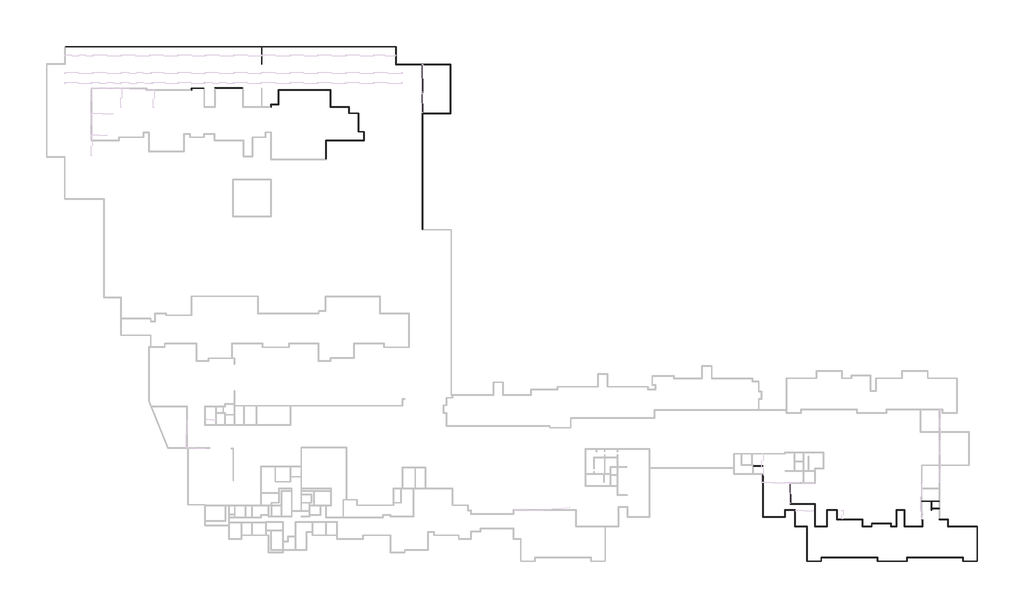
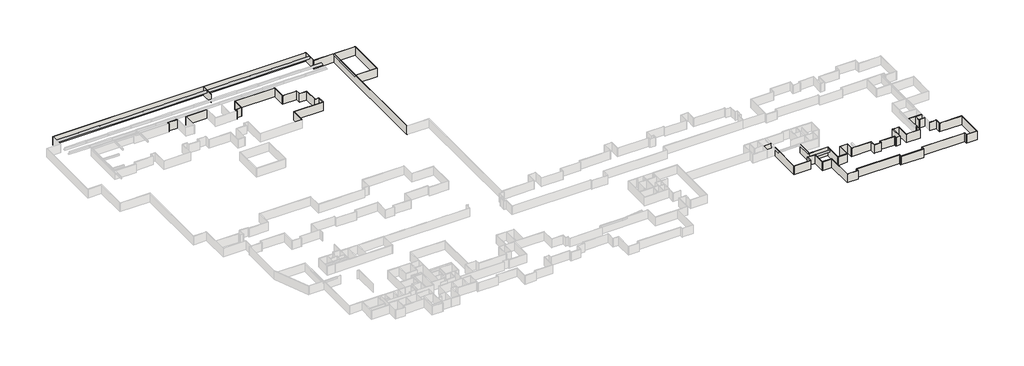
# One storey, part 6 of 8: 67 walls.
"""IFC4 building model written with IfcOpenShell, lengths in millimetres."""

from ifc_helpers import new_model, si_unit, origin, origin_with_axes, place, context, project, spatial, polyline, outline, extrude, faceted_brep, element, save

model = new_model("IFC4")

# Units and contexts
model_context = context("Model", 3, world=origin())
ifc_project = project(units=[si_unit("LENGTHUNIT", "METRE", prefix="MILLI")], contexts=[model_context])

# Site, building, storey
site = spatial("IfcSite", under=ifc_project)
building = spatial("IfcBuilding", under=site)
storey = spatial("IfcBuildingStorey", under=building, Name="户型图", Elevation=0.0)

# Walls
placement = place(None, origin())
element("IfcWall", 1, ObjectType="所有墙体", at=placement, inside=storey, context=model_context, shape_type="Brep", body=[
    faceted_brep([(258613.8534901, 37656.7427445, 0.0), (258613.8534901, 25547.5338444, 0.0), (258613.8534901, 25547.5338444, 3300.0), (258613.8534901, 37656.7427445, 3300.0), (258733.8534901, 37656.7427445, 0.0), (258733.8534901, 37656.7427445, 3300.0), (258733.8534901, 25667.5338444, 3300.0), (258733.8534901, 25547.5338444, 3300.0), (258733.8534901, 25547.5338444, 0.0), (258733.8534901, 25667.5338444, 0.0)], [[[0, 1, 2, 3]], [[4, 5, 6, 7, 8, 9]], [[1, 0, 4, 9, 8]], [[3, 2, 7, 6, 5]], [[0, 3, 5, 4]], [[2, 1, 8, 7]]]),
])
element("IfcWall", 2, ObjectType="所有墙体", at=placement, inside=storey, context=model_context, shape_type="Brep", body=[
    faceted_brep([(258733.8534901, 25547.5338444, 0.0), (264932.3033606, 25547.5338444, 0.0), (264932.3033606, 25547.5338444, 3300.0), (258733.8534901, 25547.5338444, 3300.0), (258733.8534901, 25667.5338444, 0.0), (258733.8534901, 25667.5338444, 3300.0), (264812.3033606, 25667.5338444, 3300.0), (264932.3033606, 25667.5338444, 3300.0), (264932.3033606, 25667.5338444, 0.0), (264812.3033606, 25667.5338444, 0.0)], [[[0, 1, 2, 3]], [[4, 5, 6, 7, 8, 9]], [[1, 0, 4, 9, 8]], [[3, 2, 7, 6, 5]], [[0, 3, 5, 4]], [[2, 1, 8, 7]]]),
])
element("IfcWall", 3, ObjectType="所有墙体", at=placement, inside=storey, context=model_context, shape_type="Brep", body=[
    faceted_brep([(264932.3033606, 25667.5338444, 0.0), (264932.3033606, 27556.847508, 0.0), (264932.3033606, 27676.847508, 0.0), (264932.3033606, 27676.847508, 3300.0), (264932.3033606, 27556.847508, 3300.0), (264932.3033606, 25667.5338444, 3300.0), (264812.3033606, 25667.5338444, 0.0), (264812.3033606, 25667.5338444, 3300.0), (264812.3033606, 27676.847508, 3300.0), (264812.3033606, 27676.847508, 0.0)], [[[0, 1, 2, 3, 4, 5]], [[6, 7, 8, 9]], [[2, 1, 0, 6, 9]], [[5, 4, 3, 8, 7]], [[0, 5, 7, 6]], [[3, 2, 9, 8]]]),
])
element("IfcWall", 4, ObjectType="所有墙体", at=placement, inside=storey, context=model_context, shape_type="Brep", body=[
    faceted_brep([(264932.3033606, 27556.847508, 0.0), (267613.3412105, 27556.847508, 0.0), (267733.3412105, 27556.847508, 0.0), (267733.3412105, 27556.847508, 3300.0), (267613.3412105, 27556.847508, 3300.0), (264932.3033606, 27556.847508, 3300.0), (264932.3033606, 27676.847508, 0.0), (264932.3033606, 27676.847508, 3300.0), (267733.3412105, 27676.847508, 3300.0), (267733.3412105, 27676.847508, 0.0)], [[[0, 1, 2, 3, 4, 5]], [[6, 7, 8, 9]], [[2, 1, 0, 6, 9]], [[5, 4, 3, 8, 7]], [[0, 5, 7, 6]], [[3, 2, 9, 8]]]),
])
element("IfcWall", 5, ObjectType="所有墙体", at=placement, inside=storey, context=model_context, shape_type="Brep", body=[
    faceted_brep([(267613.3412105, 27556.847508, 0.0), (267613.3412105, 22947.648549, 0.0), (267613.3412105, 22947.648549, 3300.0), (267613.3412105, 27556.847508, 3300.0), (267733.3412105, 27556.847508, 0.0), (267733.3412105, 27556.847508, 3300.0), (267733.3412105, 23067.648549, 3300.0), (267733.3412105, 22947.648549, 3300.0), (267733.3412105, 22947.648549, 0.0), (267733.3412105, 23067.648549, 0.0)], [[[0, 1, 2, 3]], [[4, 5, 6, 7, 8, 9]], [[1, 0, 4, 9, 8]], [[3, 2, 7, 6, 5]], [[0, 3, 5, 4]], [[2, 1, 8, 7]]]),
])
element("IfcWall", 6, ObjectType="所有墙体", at=placement, inside=storey, context=model_context, shape_type="Brep", body=[
    faceted_brep([(267733.3412105, 22947.648549, 0.0), (271063.0918563, 22947.648549, 0.0), (271183.0918563, 22947.648549, 0.0), (271183.0918563, 22947.648549, 3300.0), (271063.0918563, 22947.648549, 3300.0), (267733.3412105, 22947.648549, 3300.0), (267733.3412105, 23067.648549, 0.0), (267733.3412105, 23067.648549, 3300.0), (271183.0918563, 23067.648549, 3300.0), (271183.0918563, 23067.648549, 0.0)], [[[0, 1, 2, 3, 4, 5]], [[6, 7, 8, 9]], [[2, 1, 0, 6, 9]], [[5, 4, 3, 8, 7]], [[0, 5, 7, 6]], [[3, 2, 9, 8]]]),
])
element("IfcWall", 7, ObjectType="所有墙体", at=placement, inside=storey, context=model_context, shape_type="Brep", body=[
    faceted_brep([(271063.0918563, 22947.648549, 0.0), (271063.0918563, 13147.6884452, 0.0), (271063.0918563, 13147.6884452, 3300.0), (271063.0918563, 22947.648549, 3300.0), (271183.0918563, 22947.648549, 0.0), (271183.0918563, 22947.648549, 3300.0), (271183.0918563, 13267.6884452, 3300.0), (271183.0918563, 13147.6884452, 3300.0), (271183.0918563, 13147.6884452, 0.0), (271183.0918563, 13267.6884452, 0.0)], [[[0, 1, 2, 3]], [[4, 5, 6, 7, 8, 9]], [[1, 0, 4, 9, 8]], [[3, 2, 7, 6, 5]], [[0, 3, 5, 4]], [[2, 1, 8, 7]]]),
])
element("IfcWall", 8, ObjectType="所有墙体", at=placement, inside=storey, context=model_context, shape_type="Brep", body=[
    faceted_brep([(271183.0918563, 13147.6884452, 0.0), (275183.1173563, 13147.6884452, 0.0), (275183.1173563, 13147.6884452, 3300.0), (271183.0918563, 13147.6884452, 3300.0), (271183.0918563, 13267.6884452, 0.0), (271183.0918563, 13267.6884452, 3300.0), (275063.1173563, 13267.6884452, 3300.0), (275183.1173563, 13267.6884452, 3300.0), (275183.1173563, 13267.6884452, 0.0), (275063.1173563, 13267.6884452, 0.0)], [[[0, 1, 2, 3]], [[4, 5, 6, 7, 8, 9]], [[1, 0, 4, 9, 8]], [[3, 2, 7, 6, 5]], [[0, 3, 5, 4]], [[2, 1, 8, 7]]]),
])
element("IfcWall", 9, ObjectType="所有墙体", at=placement, inside=storey, context=model_context, shape_type="Brep", body=[
    faceted_brep([(275183.1173563, 13267.6884452, 0.0), (275183.1173563, 14147.2784493, 0.0), (275183.1173563, 14267.2784493, 0.0), (275183.1173563, 14267.2784493, 3300.0), (275183.1173563, 14147.2784493, 3300.0), (275183.1173563, 13267.6884452, 3300.0), (275063.1173563, 13267.6884452, 0.0), (275063.1173563, 13267.6884452, 3300.0), (275063.1173563, 14267.2784493, 3300.0), (275063.1173563, 14267.2784493, 0.0)], [[[0, 1, 2, 3, 4, 5]], [[6, 7, 8, 9]], [[2, 1, 0, 6, 9]], [[5, 4, 3, 8, 7]], [[0, 5, 7, 6]], [[3, 2, 9, 8]]]),
])
element("IfcWall", 10, ObjectType="所有墙体", at=placement, inside=storey, context=model_context, shape_type="Brep", body=[
    faceted_brep([(275183.1173563, 14147.2784493, 0.0), (290862.8910266, 14147.2784493, 0.0), (290982.8910266, 14147.2784493, 0.0), (290982.8910266, 14147.2784493, 3300.0), (290862.8910266, 14147.2784493, 3300.0), (275183.1173563, 14147.2784493, 3300.0), (275183.1173563, 14267.2784493, 0.0), (275183.1173563, 14267.2784493, 3300.0), (290982.8910266, 14267.2784493, 3300.0), (290982.8910266, 14267.2784493, 0.0)], [[[0, 1, 2, 3, 4, 5]], [[6, 7, 8, 9]], [[2, 1, 0, 6, 9]], [[5, 4, 3, 8, 7]], [[0, 5, 7, 6]], [[3, 2, 9, 8]]]),
])
element("IfcWall", 11, ObjectType="所有墙体", at=placement, inside=storey, context=model_context, shape_type="Brep", body=[
    faceted_brep([(290862.8910266, 14147.2784493, 0.0), (290862.8910266, 13147.6884452, 0.0), (290862.8910266, 13147.6884452, 3300.0), (290862.8910266, 14147.2784493, 3300.0), (290982.8910266, 14147.2784493, 0.0), (290982.8910266, 14147.2784493, 3300.0), (290982.8910266, 13267.6884452, 3300.0), (290982.8910266, 13147.6884452, 3300.0), (290982.8910266, 13147.6884452, 0.0), (290982.8910266, 13267.6884452, 0.0)], [[[0, 1, 2, 3]], [[4, 5, 6, 7, 8, 9]], [[1, 0, 4, 9, 8]], [[3, 2, 7, 6, 5]], [[0, 3, 5, 4]], [[2, 1, 8, 7]]]),
])
element("IfcWall", 12, ObjectType="所有墙体", at=placement, inside=storey, context=model_context, shape_type="Brep", body=[
    faceted_brep([(290982.8910266, 13147.6884452, 0.0), (299283.1811417, 13147.6884452, 0.0), (299283.1811417, 13147.6884452, 3300.0), (290982.8910266, 13147.6884452, 3300.0), (290982.8910266, 13267.6884452, 0.0), (290982.8910266, 13267.6884452, 3300.0), (299163.1811417, 13267.6884452, 3300.0), (299283.1811417, 13267.6884452, 3300.0), (299283.1811417, 13267.6884452, 0.0), (299163.1811417, 13267.6884452, 0.0)], [[[0, 1, 2, 3]], [[4, 5, 6, 7, 8, 9]], [[1, 0, 4, 9, 8]], [[3, 2, 7, 6, 5]], [[0, 3, 5, 4]], [[2, 1, 8, 7]]]),
])
element("IfcWall", 13, ObjectType="所有墙体", at=placement, inside=storey, context=model_context, shape_type="Brep", body=[
    faceted_brep([(299283.1811417, 13267.6884452, 0.0), (299283.1811417, 14147.2784493, 0.0), (299283.1811417, 14267.2784493, 0.0), (299283.1811417, 14267.2784493, 3300.0), (299283.1811417, 14147.2784493, 3300.0), (299283.1811417, 13267.6884452, 3300.0), (299163.1811417, 13267.6884452, 0.0), (299163.1811417, 13267.6884452, 3300.0), (299163.1811417, 14267.2784493, 3300.0), (299163.1811417, 14267.2784493, 0.0)], [[[0, 1, 2, 3, 4, 5]], [[6, 7, 8, 9]], [[2, 1, 0, 6, 9]], [[5, 4, 3, 8, 7]], [[0, 5, 7, 6]], [[3, 2, 9, 8]]]),
])
element("IfcWall", 14, ObjectType="所有墙体", at=placement, inside=storey, context=model_context, shape_type="Brep", body=[
    faceted_brep([(299283.1811417, 14147.2784493, 0.0), (314962.8909977, 14147.2784493, 0.0), (315082.8909977, 14147.2784493, 0.0), (315082.8909977, 14147.2784493, 3300.0), (314962.8909977, 14147.2784493, 3300.0), (299283.1811417, 14147.2784493, 3300.0), (299283.1811417, 14267.2784493, 0.0), (299283.1811417, 14267.2784493, 3300.0), (315082.8909977, 14267.2784493, 3300.0), (315082.8909977, 14267.2784493, 0.0)], [[[0, 1, 2, 3, 4, 5]], [[6, 7, 8, 9]], [[2, 1, 0, 6, 9]], [[5, 4, 3, 8, 7]], [[0, 5, 7, 6]], [[3, 2, 9, 8]]]),
])
element("IfcWall", 15, ObjectType="所有墙体", at=placement, inside=storey, context=model_context, shape_type="Brep", body=[
    faceted_brep([(314962.8909977, 14147.2784493, 0.0), (314962.8909977, 13147.6884452, 0.0), (314962.8909977, 13147.6884452, 3300.0), (314962.8909977, 14147.2784493, 3300.0), (315082.8909977, 14147.2784493, 0.0), (315082.8909977, 14147.2784493, 3300.0), (315082.8909977, 13267.6884452, 3300.0), (315082.8909977, 13147.6884452, 3300.0), (315082.8909977, 13147.6884452, 0.0), (315082.8909977, 13267.6884452, 0.0)], [[[0, 1, 2, 3]], [[4, 5, 6, 7, 8, 9]], [[1, 0, 4, 9, 8]], [[3, 2, 7, 6, 5]], [[0, 3, 5, 4]], [[2, 1, 8, 7]]]),
])
element("IfcWall", 16, ObjectType="所有墙体", at=placement, inside=storey, context=model_context, shape_type="Brep", body=[
    faceted_brep([(315082.8909977, 13147.6884452, 0.0), (319083.2156356, 13147.6884452, 0.0), (319083.2156356, 13147.6884452, 3300.0), (315082.8909977, 13147.6884452, 3300.0), (315082.8909977, 13267.6884452, 0.0), (315082.8909977, 13267.6884452, 3300.0), (318963.2156356, 13267.6884452, 3300.0), (319083.2156356, 13267.6884452, 3300.0), (319083.2156356, 13267.6884452, 0.0), (318963.2156356, 13267.6884452, 0.0)], [[[0, 1, 2, 3]], [[4, 5, 6, 7, 8, 9]], [[1, 0, 4, 9, 8]], [[3, 2, 7, 6, 5]], [[0, 3, 5, 4]], [[2, 1, 8, 7]]]),
])
element("IfcWall", 17, ObjectType="所有墙体", at=placement, inside=storey, context=model_context, shape_type="Brep", body=[
    faceted_brep([(319083.2156356, 13267.6884452, 0.0), (319083.2156356, 23067.648549, 0.0), (319083.2156356, 23067.648549, 3300.0), (319083.2156356, 13267.6884452, 3300.0), (318963.2156356, 13267.6884452, 0.0), (318963.2156356, 13267.6884452, 3300.0), (318963.2156356, 22947.648549, 3300.0), (318963.2156356, 23067.648549, 3300.0), (318963.2156356, 23067.648549, 0.0), (318963.2156356, 22947.648549, 0.0)], [[[0, 1, 2, 3]], [[4, 5, 6, 7, 8, 9]], [[1, 0, 4, 9, 8]], [[3, 2, 7, 6, 5]], [[0, 3, 5, 4]], [[2, 1, 8, 7]]]),
])
element("IfcWall", 18, ObjectType="所有墙体", at=placement, inside=storey, context=model_context, shape_type="Brep", body=[
    faceted_brep([(318963.2156356, 23067.648549, 0.0), (310883.5691593, 23067.648549, 0.0), (310763.5691593, 23067.648549, 0.0), (310763.5691593, 23067.648549, 3300.0), (310883.5691593, 23067.648549, 3300.0), (318963.2156356, 23067.648549, 3300.0), (318963.2156356, 22947.648549, 0.0), (318963.2156356, 22947.648549, 3300.0), (310763.5691593, 22947.648549, 3300.0), (310763.5691593, 22947.648549, 0.0)], [[[0, 1, 2, 3, 4, 5]], [[6, 7, 8, 9]], [[2, 1, 0, 6, 9]], [[5, 4, 3, 8, 7]], [[0, 5, 7, 6]], [[3, 2, 9, 8]]]),
])
element("IfcWall", 19, ObjectType="所有墙体", at=placement, inside=storey, context=model_context, shape_type="Brep", body=[
    faceted_brep([(310883.5691593, 23067.648549, 0.0), (310883.5691593, 25066.2785565, 0.0), (310883.5691593, 25066.2785565, 3300.0), (310883.5691593, 23067.648549, 3300.0), (310763.5691593, 23067.648549, 0.0), (310763.5691593, 23067.648549, 3300.0), (310763.5691593, 24946.2785565, 3300.0), (310763.5691593, 25066.2785565, 3300.0), (310763.5691593, 25066.2785565, 0.0), (310763.5691593, 24946.2785565, 0.0)], [[[0, 1, 2, 3]], [[4, 5, 6, 7, 8, 9]], [[1, 0, 4, 9, 8]], [[3, 2, 7, 6, 5]], [[0, 3, 5, 4]], [[2, 1, 8, 7]]]),
])
element("IfcWall", 20, ObjectType="所有墙体", at=placement, inside=storey, context=model_context, shape_type="Brep", body=[
    faceted_brep([(310763.5691593, 25066.2785565, 0.0), (308483.5691593, 25066.2785565, 0.0), (308363.5691593, 25066.2785565, 0.0), (308363.5691593, 25066.2785565, 3300.0), (308483.5691593, 25066.2785565, 3300.0), (310763.5691593, 25066.2785565, 3300.0), (310763.5691593, 24946.2785565, 0.0), (310763.5691593, 24946.2785565, 3300.0), (308363.5691593, 24946.2785565, 3300.0), (308363.5691593, 24946.2785565, 0.0)], [[[0, 1, 2, 3, 4, 5]], [[6, 7, 8, 9]], [[2, 1, 0, 6, 9]], [[5, 4, 3, 8, 7]], [[0, 5, 7, 6]], [[3, 2, 9, 8]]]),
])
element("IfcWall", 21, ObjectType="所有墙体", at=placement, inside=storey, context=model_context, shape_type="Brep", body=[
    faceted_brep([(162933.8477327, 106576.635667, 0.0), (162933.8477327, 139156.635667, 0.0), (162933.8477327, 139276.635667, 0.0), (162933.8477327, 153006.6496336, 0.0), (162933.8477327, 153006.6496336, 3300.0), (162933.8477327, 139276.635667, 3300.0), (162933.8477327, 139156.635667, 3300.0), (162933.8477327, 106576.635667, 3300.0), (162813.8477327, 106576.635667, 0.0), (162813.8477327, 106576.635667, 3300.0), (162813.8477327, 153006.6496336, 3300.0), (162813.8477327, 153006.6496336, 0.0)], [[[0, 1, 2, 3, 4, 5, 6, 7]], [[8, 9, 10, 11]], [[3, 2, 1, 0, 8, 11]], [[7, 6, 5, 4, 10, 9]], [[0, 7, 9, 8]], [[4, 3, 11, 10]]]),
])
element("IfcWall", 22, ObjectType="所有墙体", at=placement, inside=storey, context=model_context, shape_type="Brep", body=[
    faceted_brep([(162933.8477327, 139156.635667, 0.0), (170833.8477327, 139156.635667, 0.0), (170833.8477327, 139156.635667, 3300.0), (162933.8477327, 139156.635667, 3300.0), (162933.8477327, 139276.635667, 0.0), (162933.8477327, 139276.635667, 3300.0), (170713.8477327, 139276.635667, 3300.0), (170833.8477327, 139276.635667, 3300.0), (170833.8477327, 139276.635667, 0.0), (170713.8477327, 139276.635667, 0.0)], [[[0, 1, 2, 3]], [[4, 5, 6, 7, 8, 9]], [[1, 0, 4, 9, 8]], [[3, 2, 7, 6, 5]], [[0, 3, 5, 4]], [[2, 1, 8, 7]]]),
])
element("IfcWall", 23, ObjectType="所有墙体", at=placement, inside=storey, context=model_context, shape_type="Brep", body=[
    faceted_brep([(170833.8477327, 139276.635667, 0.0), (170833.8477327, 153126.6496336, 0.0), (170833.8477327, 153126.6496336, 3300.0), (170833.8477327, 139276.635667, 3300.0), (170713.8477327, 139276.635667, 0.0), (170713.8477327, 139276.635667, 3300.0), (170713.8477327, 153006.6496336, 3300.0), (170713.8477327, 153126.6496336, 3300.0), (170713.8477327, 153126.6496336, 0.0), (170713.8477327, 153006.6496336, 0.0)], [[[0, 1, 2, 3]], [[4, 5, 6, 7, 8, 9]], [[1, 0, 4, 9, 8]], [[3, 2, 7, 6, 5]], [[0, 3, 5, 4]], [[2, 1, 8, 7]]]),
])
element("IfcWall", 24, ObjectType="所有墙体", at=placement, inside=storey, context=model_context, shape_type="Brep", body=[
    faceted_brep([(170713.8477327, 153126.6496336, 0.0), (155458.8476291, 153126.6496336, 0.0), (155338.8476291, 153126.6496336, 0.0), (155338.8476291, 153126.6496336, 3300.0), (155458.8476291, 153126.6496336, 3300.0), (170713.8477327, 153126.6496336, 3300.0), (170713.8477327, 153006.6496336, 0.0), (170713.8477327, 153006.6496336, 3300.0), (162933.8477327, 153006.6496336, 3300.0), (162813.8477327, 153006.6496336, 3300.0), (155338.8476291, 153006.6496336, 3300.0), (155338.8476291, 153006.6496336, 0.0), (162813.8477327, 153006.6496336, 0.0), (162933.8477327, 153006.6496336, 0.0)], [[[0, 1, 2, 3, 4, 5]], [[6, 7, 8, 9, 10, 11, 12, 13]], [[2, 1, 0, 6, 13, 12, 11]], [[5, 4, 3, 10, 9, 8, 7]], [[0, 5, 7, 6]], [[3, 2, 11, 10]]]),
])
element("IfcWall", 25, ObjectType="所有墙体", at=placement, inside=storey, context=model_context, shape_type="Brep", body=[
    faceted_brep([(155458.8476291, 153126.6496336, 0.0), (155458.8476291, 158076.8472847, 0.0), (155458.8476291, 158076.8472847, 3300.0), (155458.8476291, 153126.6496336, 3300.0), (155338.8476291, 153126.6496336, 0.0), (155338.8476291, 153126.6496336, 3300.0), (155338.8476291, 157956.8472847, 3300.0), (155338.8476291, 158076.8472847, 3300.0), (155338.8476291, 158076.8472847, 0.0), (155338.8476291, 157956.8472847, 0.0)], [[[0, 1, 2, 3]], [[4, 5, 6, 7, 8, 9]], [[1, 0, 4, 9, 8]], [[3, 2, 7, 6, 5]], [[0, 3, 5, 4]], [[2, 1, 8, 7]]]),
])
element("IfcWall", 26, ObjectType="所有墙体", at=placement, inside=storey, context=model_context, shape_type="Brep", body=[
    faceted_brep([(155338.8476291, 158076.8472847, 0.0), (62138.8476291, 158076.8472847, 0.0), (62138.8476291, 158076.8472847, 3300.0), (155338.8476291, 158076.8472847, 3300.0), (155338.8476291, 157956.8472847, 0.0), (155338.8476291, 157956.8472847, 3300.0), (117696.3185581, 157956.8472847, 3300.0), (117576.3185581, 157956.8472847, 3300.0), (62258.8476291, 157956.8472847, 3300.0), (62138.8476291, 157956.8472847, 3300.0), (62138.8476291, 157956.8472847, 0.0), (62258.8476291, 157956.8472847, 0.0), (117576.3185581, 157956.8472847, 0.0), (117696.3185581, 157956.8472847, 0.0)], [[[0, 1, 2, 3]], [[4, 5, 6, 7, 8, 9, 10, 11, 12, 13]], [[1, 0, 4, 13, 12, 11, 10]], [[3, 2, 9, 8, 7, 6, 5]], [[0, 3, 5, 4]], [[2, 1, 10, 9]]]),
])
element("IfcWall", 27, ObjectType="所有墙体", at=placement, inside=storey, context=model_context, shape_type="Brep", body=[
    faceted_brep([(135753.7737349, 126356.2446076, 0.0), (135753.7737349, 131533.7456111, 0.0), (135753.7737349, 131653.7456111, 0.0), (135753.7737349, 131653.7456111, 3300.0), (135753.7737349, 131533.7456111, 3300.0), (135753.7737349, 126356.2446076, 3300.0), (135633.7737349, 126356.2446076, 0.0), (135633.7737349, 126356.2446076, 3300.0), (135633.7737349, 131653.7456111, 3300.0), (135633.7737349, 131653.7456111, 0.0)], [[[0, 1, 2, 3, 4, 5]], [[6, 7, 8, 9]], [[2, 1, 0, 6, 9]], [[5, 4, 3, 8, 7]], [[0, 5, 7, 6]], [[3, 2, 9, 8]]]),
])
element("IfcWall", 28, ObjectType="所有墙体", at=placement, inside=storey, context=model_context, shape_type="Brep", body=[
    faceted_brep([(135753.7737349, 131533.7456111, 0.0), (146453.7737349, 131533.7456111, 0.0), (146453.7737349, 131533.7456111, 3300.0), (135753.7737349, 131533.7456111, 3300.0), (135753.7737349, 131653.7456111, 0.0), (135753.7737349, 131653.7456111, 3300.0), (146333.7737349, 131653.7456111, 3300.0), (146453.7737349, 131653.7456111, 3300.0), (146453.7737349, 131653.7456111, 0.0), (146333.7737349, 131653.7456111, 0.0)], [[[0, 1, 2, 3]], [[4, 5, 6, 7, 8, 9]], [[1, 0, 4, 9, 8]], [[3, 2, 7, 6, 5]], [[0, 3, 5, 4]], [[2, 1, 8, 7]]]),
])
element("IfcWall", 29, ObjectType="所有墙体", at=placement, inside=storey, context=model_context, shape_type="Brep", body=[
    faceted_brep([(146453.7737349, 131653.7456111, 0.0), (146453.7737349, 134154.479138, 0.0), (146453.7737349, 134154.479138, 3300.0), (146453.7737349, 131653.7456111, 3300.0), (146333.7737349, 131653.7456111, 0.0), (146333.7737349, 131653.7456111, 3300.0), (146333.7737349, 134034.479138, 3300.0), (146333.7737349, 134154.479138, 3300.0), (146333.7737349, 134154.479138, 0.0), (146333.7737349, 134034.479138, 0.0)], [[[0, 1, 2, 3]], [[4, 5, 6, 7, 8, 9]], [[1, 0, 4, 9, 8]], [[3, 2, 7, 6, 5]], [[0, 3, 5, 4]], [[2, 1, 8, 7]]]),
])
element("IfcWall", 30, ObjectType="所有墙体", at=placement, inside=storey, context=model_context, shape_type="Brep", body=[
    faceted_brep([(146333.7737349, 134154.479138, 0.0), (144953.4366403, 134154.479138, 0.0), (144833.4366403, 134154.479138, 0.0), (144833.4366403, 134154.479138, 3300.0), (144953.4366403, 134154.479138, 3300.0), (146333.7737349, 134154.479138, 3300.0), (146333.7737349, 134034.479138, 0.0), (146333.7737349, 134034.479138, 3300.0), (144833.4366403, 134034.479138, 3300.0), (144833.4366403, 134034.479138, 0.0)], [[[0, 1, 2, 3, 4, 5]], [[6, 7, 8, 9]], [[2, 1, 0, 6, 9]], [[5, 4, 3, 8, 7]], [[0, 5, 7, 6]], [[3, 2, 9, 8]]]),
])
element("IfcWall", 31, ObjectType="所有墙体", at=placement, inside=storey, context=model_context, shape_type="Brep", body=[
    faceted_brep([(144953.4366403, 134154.479138, 0.0), (144953.4366403, 139354.4795445, 0.0), (144953.4366403, 139354.4795445, 3300.0), (144953.4366403, 134154.479138, 3300.0), (144833.4366403, 134154.479138, 0.0), (144833.4366403, 134154.479138, 3300.0), (144833.4366403, 139234.4795445, 3300.0), (144833.4366403, 139354.4795445, 3300.0), (144833.4366403, 139354.4795445, 0.0), (144833.4366403, 139234.4795445, 0.0)], [[[0, 1, 2, 3]], [[4, 5, 6, 7, 8, 9]], [[1, 0, 4, 9, 8]], [[3, 2, 7, 6, 5]], [[0, 3, 5, 4]], [[2, 1, 8, 7]]]),
])
element("IfcWall", 32, ObjectType="所有墙体", at=placement, inside=storey, context=model_context, shape_type="Brep", body=[
    faceted_brep([(144833.4366403, 139354.4795445, 0.0), (142253.4366403, 139354.4795445, 0.0), (142133.4366403, 139354.4795445, 0.0), (142133.4366403, 139354.4795445, 3300.0), (142253.4366403, 139354.4795445, 3300.0), (144833.4366403, 139354.4795445, 3300.0), (144833.4366403, 139234.4795445, 0.0), (144833.4366403, 139234.4795445, 3300.0), (142133.4366403, 139234.4795445, 3300.0), (142133.4366403, 139234.4795445, 0.0)], [[[0, 1, 2, 3, 4, 5]], [[6, 7, 8, 9]], [[2, 1, 0, 6, 9]], [[5, 4, 3, 8, 7]], [[0, 5, 7, 6]], [[3, 2, 9, 8]]]),
])
element("IfcWall", 33, ObjectType="所有墙体", at=placement, inside=storey, context=model_context, shape_type="Brep", body=[
    faceted_brep([(142253.4366403, 139354.4795445, 0.0), (142253.4366403, 141065.2964279, 0.0), (142253.4366403, 141065.2964279, 3300.0), (142253.4366403, 139354.4795445, 3300.0), (142133.4366403, 139354.4795445, 0.0), (142133.4366403, 139354.4795445, 3300.0), (142133.4366403, 140945.2964279, 3300.0), (142133.4366403, 141065.2964279, 3300.0), (142133.4366403, 141065.2964279, 0.0), (142133.4366403, 140945.2964279, 0.0)], [[[0, 1, 2, 3]], [[4, 5, 6, 7, 8, 9]], [[1, 0, 4, 9, 8]], [[3, 2, 7, 6, 5]], [[0, 3, 5, 4]], [[2, 1, 8, 7]]]),
])
element("IfcWall", 34, ObjectType="所有墙体", at=placement, inside=storey, context=model_context, shape_type="Brep", body=[
    faceted_brep([(142133.4366403, 141065.2964279, 0.0), (137052.6046447, 141065.2964279, 0.0), (136932.6046447, 141065.2964279, 0.0), (136932.6046447, 141065.2964279, 3300.0), (137052.6046447, 141065.2964279, 3300.0), (142133.4366403, 141065.2964279, 3300.0), (142133.4366403, 140945.2964279, 0.0), (142133.4366403, 140945.2964279, 3300.0), (136932.6046447, 140945.2964279, 3300.0), (136932.6046447, 140945.2964279, 0.0)], [[[0, 1, 2, 3, 4, 5]], [[6, 7, 8, 9]], [[2, 1, 0, 6, 9]], [[5, 4, 3, 8, 7]], [[0, 5, 7, 6]], [[3, 2, 9, 8]]]),
])
element("IfcWall", 35, ObjectType="所有墙体", at=placement, inside=storey, context=model_context, shape_type="Brep", body=[
    faceted_brep([(137052.6046447, 141065.2964279, 0.0), (137052.6046447, 145945.2964279, 0.0), (137052.6046447, 145945.2964279, 3300.0), (137052.6046447, 141065.2964279, 3300.0), (136932.6046447, 141065.2964279, 0.0), (136932.6046447, 141065.2964279, 3300.0), (136932.6046447, 145825.2964279, 3300.0), (136932.6046447, 145945.2964279, 3300.0), (136932.6046447, 145945.2964279, 0.0), (136932.6046447, 145825.2964279, 0.0)], [[[0, 1, 2, 3]], [[4, 5, 6, 7, 8, 9]], [[1, 0, 4, 9, 8]], [[3, 2, 7, 6, 5]], [[0, 3, 5, 4]], [[2, 1, 8, 7]]]),
])
element("IfcWall", 36, ObjectType="所有墙体", at=placement, inside=storey, context=model_context, shape_type="Brep", body=[
    faceted_brep([(136932.6046447, 145945.2964279, 0.0), (122272.6046447, 145945.2964279, 0.0), (122272.6046447, 145945.2964279, 3300.0), (136932.6046447, 145945.2964279, 3300.0), (136932.6046447, 145825.2964279, 0.0), (136932.6046447, 145825.2964279, 3300.0), (122392.6046447, 145825.2964279, 3300.0), (122272.6046447, 145825.2964279, 3300.0), (122272.6046447, 145825.2964279, 0.0), (122392.6046447, 145825.2964279, 0.0)], [[[0, 1, 2, 3]], [[4, 5, 6, 7, 8, 9]], [[1, 0, 4, 9, 8]], [[3, 2, 7, 6, 5]], [[0, 3, 5, 4]], [[2, 1, 8, 7]]]),
])
element("IfcWall", 37, ObjectType="所有墙体", at=placement, inside=storey, context=model_context, shape_type="Brep", body=[
    faceted_brep([(122272.6046447, 145825.2964279, 0.0), (122272.6046447, 141845.2964279, 0.0), (122272.6046447, 141725.2964279, 0.0), (122272.6046447, 141725.2964279, 3300.0), (122272.6046447, 141845.2964279, 3300.0), (122272.6046447, 145825.2964279, 3300.0), (122392.6046447, 145825.2964279, 0.0), (122392.6046447, 145825.2964279, 3300.0), (122392.6046447, 141725.2964279, 3300.0), (122392.6046447, 141725.2964279, 0.0)], [[[0, 1, 2, 3, 4, 5]], [[6, 7, 8, 9]], [[2, 1, 0, 6, 9]], [[5, 4, 3, 8, 7]], [[0, 5, 7, 6]], [[3, 2, 9, 8]]]),
])
element("IfcWall", 38, ObjectType="所有墙体", at=placement, inside=storey, context=model_context, shape_type="Brep", body=[
    faceted_brep([(122272.6046447, 141845.2964279, 0.0), (120182.8546857, 141845.2964279, 0.0), (120182.8546857, 141845.2964279, 3300.0), (122272.6046447, 141845.2964279, 3300.0), (122272.6046447, 141725.2964279, 0.0), (122272.6046447, 141725.2964279, 3300.0), (120302.8546857, 141725.2964279, 3300.0), (120182.8546857, 141725.2964279, 3300.0), (120182.8546857, 141725.2964279, 0.0), (120302.8546857, 141725.2964279, 0.0)], [[[0, 1, 2, 3]], [[4, 5, 6, 7, 8, 9]], [[1, 0, 4, 9, 8]], [[3, 2, 7, 6, 5]], [[0, 3, 5, 4]], [[2, 1, 8, 7]]]),
])
element("IfcWall", 39, ObjectType="所有墙体", at=placement, inside=storey, context=model_context, shape_type="Brep", body=[
    faceted_brep([(120182.8546857, 141725.2964279, 0.0), (120182.8546857, 141104.2446487, 0.0), (120182.8546857, 140984.2446487, 0.0), (120182.8546857, 140984.2446487, 3300.0), (120182.8546857, 141104.2446487, 3300.0), (120182.8546857, 141725.2964279, 3300.0), (120302.8546857, 141725.2964279, 0.0), (120302.8546857, 141725.2964279, 3300.0), (120302.8546857, 140984.2446487, 3300.0), (120302.8546857, 140984.2446487, 0.0)], [[[0, 1, 2, 3, 4, 5]], [[6, 7, 8, 9]], [[2, 1, 0, 6, 9]], [[5, 4, 3, 8, 7]], [[0, 5, 7, 6]], [[3, 2, 9, 8]]]),
])
element("IfcWall", 40, ObjectType="所有墙体", at=placement, inside=storey, context=model_context, shape_type="Brep", body=[
    faceted_brep([(112238.82396, 146454.2446479, 0.0), (104388.8715153, 146454.2446479, 0.0), (104388.8715153, 146454.2446479, 3300.0), (112238.82396, 146454.2446479, 3300.0), (112238.82396, 146334.2446479, 0.0), (112238.82396, 146334.2446479, 3300.0), (104508.8715153, 146334.2446479, 3300.0), (104388.8715153, 146334.2446479, 3300.0), (104388.8715153, 146334.2446479, 0.0), (104508.8715153, 146334.2446479, 0.0)], [[[0, 1, 2, 3]], [[4, 5, 6, 7, 8, 9]], [[1, 0, 4, 9, 8]], [[3, 2, 7, 6, 5]], [[0, 3, 5, 4]], [[2, 1, 8, 7]]]),
])
element("IfcWall", 41, ObjectType="所有墙体", at=placement, inside=storey, context=model_context, shape_type="Brep", body=[
    faceted_brep([(101372.8755148, 146404.244647, 0.0), (97832.8755148, 146404.244647, 0.0), (97832.8755148, 146404.244647, 3300.0), (101372.8755148, 146404.244647, 3300.0), (101372.8755148, 146284.244647, 0.0), (101372.8755148, 146284.244647, 3300.0), (97952.8755148, 146284.244647, 3300.0), (97832.8755148, 146284.244647, 3300.0), (97832.8755148, 146284.244647, 0.0), (97952.8755148, 146284.244647, 0.0)], [[[0, 1, 2, 3]], [[4, 5, 6, 7, 8, 9]], [[1, 0, 4, 9, 8]], [[3, 2, 7, 6, 5]], [[0, 3, 5, 4]], [[2, 1, 8, 7]]]),
])
element("IfcWall", 42, ObjectType="所有墙体", at=placement, inside=storey, context=model_context, shape_type="Brep", body=[
    faceted_brep([(97832.8755148, 146284.244647, 0.0), (97832.8755148, 145903.9951293, 0.0), (97832.8755148, 145783.9951293, 0.0), (97832.8755148, 145783.9951293, 3300.0), (97832.8755148, 145903.9951293, 3300.0), (97832.8755148, 146284.244647, 3300.0), (97952.8755148, 146284.244647, 0.0), (97952.8755148, 146284.244647, 3300.0), (97952.8755148, 145783.9951293, 3300.0), (97952.8755148, 145783.9951293, 0.0)], [[[0, 1, 2, 3, 4, 5]], [[6, 7, 8, 9]], [[2, 1, 0, 6, 9]], [[5, 4, 3, 8, 7]], [[0, 5, 7, 6]], [[3, 2, 9, 8]]]),
])
element("IfcWall", 43, ObjectType="所有墙体", at=placement, inside=storey, context=model_context, shape_type="Brep", body=[
    faceted_brep([(266363.353082, 35106.5508771, 0.0), (266363.353082, 29206.8475027, 0.0), (266363.353082, 29206.8475027, 3300.0), (266363.353082, 35106.5508771, 3300.0), (266483.353082, 35106.5508771, 0.0), (266483.353082, 35106.5508771, 3300.0), (266483.353082, 29326.8475027, 3300.0), (266483.353082, 29206.8475027, 3300.0), (266483.353082, 29206.8475027, 0.0), (266483.353082, 29326.8475027, 0.0)], [[[0, 1, 2, 3]], [[4, 5, 6, 7, 8, 9]], [[1, 0, 4, 9, 8]], [[3, 2, 7, 6, 5]], [[0, 3, 5, 4]], [[2, 1, 8, 7]]]),
])
element("IfcWall", 44, ObjectType="所有墙体", at=placement, inside=storey, context=model_context, shape_type="Brep", body=[
    faceted_brep([(266483.353082, 29206.8475027, 0.0), (273288.1652502, 29206.8475027, 0.0), (273408.1652502, 29206.8475027, 0.0), (273408.1652502, 29206.8475027, 3300.0), (273288.1652502, 29206.8475027, 3300.0), (266483.353082, 29206.8475027, 3300.0), (266483.353082, 29326.8475027, 0.0), (266483.353082, 29326.8475027, 3300.0), (273408.1652502, 29326.8475027, 3300.0), (273408.1652502, 29326.8475027, 0.0)], [[[0, 1, 2, 3, 4, 5]], [[6, 7, 8, 9]], [[2, 1, 0, 6, 9]], [[5, 4, 3, 8, 7]], [[0, 5, 7, 6]], [[3, 2, 9, 8]]]),
])
element("IfcWall", 45, ObjectType="所有墙体", at=placement, inside=storey, context=model_context, shape_type="Brep", body=[
    faceted_brep([(273288.1652502, 29206.8475027, 0.0), (273288.1652502, 22947.648549, 0.0), (273288.1652502, 22947.648549, 3300.0), (273288.1652502, 29206.8475027, 3300.0), (273408.1652502, 29206.8475027, 0.0), (273408.1652502, 29206.8475027, 3300.0), (273408.1652502, 23067.648549, 3300.0), (273408.1652502, 22947.648549, 3300.0), (273408.1652502, 22947.648549, 0.0), (273408.1652502, 23067.648549, 0.0)], [[[0, 1, 2, 3]], [[4, 5, 6, 7, 8, 9]], [[1, 0, 4, 9, 8]], [[3, 2, 7, 6, 5]], [[0, 3, 5, 4]], [[2, 1, 8, 7]]]),
])
element("IfcWall", 46, ObjectType="所有墙体", at=placement, inside=storey, context=model_context, shape_type="Brep", body=[
    faceted_brep([(273408.1652502, 22947.648549, 0.0), (276783.4570824, 22947.648549, 0.0), (276783.4570824, 22947.648549, 3300.0), (273408.1652502, 22947.648549, 3300.0), (273408.1652502, 23067.648549, 0.0), (273408.1652502, 23067.648549, 3300.0), (276663.4570824, 23067.648549, 3300.0), (276783.4570824, 23067.648549, 3300.0), (276783.4570824, 23067.648549, 0.0), (276663.4570824, 23067.648549, 0.0)], [[[0, 1, 2, 3]], [[4, 5, 6, 7, 8, 9]], [[1, 0, 4, 9, 8]], [[3, 2, 7, 6, 5]], [[0, 3, 5, 4]], [[2, 1, 8, 7]]]),
])
element("IfcWall", 47, ObjectType="所有墙体", at=placement, inside=storey, context=model_context, shape_type="Brep", body=[
    faceted_brep([(276783.4570824, 23067.648549, 0.0), (276783.4570824, 27556.847508, 0.0), (276783.4570824, 27676.847508, 0.0), (276783.4570824, 27676.847508, 3300.0), (276783.4570824, 27556.847508, 3300.0), (276783.4570824, 23067.648549, 3300.0), (276663.4570824, 23067.648549, 0.0), (276663.4570824, 23067.648549, 3300.0), (276663.4570824, 27676.847508, 3300.0), (276663.4570824, 27676.847508, 0.0)], [[[0, 1, 2, 3, 4, 5]], [[6, 7, 8, 9]], [[2, 1, 0, 6, 9]], [[5, 4, 3, 8, 7]], [[0, 5, 7, 6]], [[3, 2, 9, 8]]]),
])
element("IfcWall", 48, ObjectType="所有墙体", at=placement, inside=storey, context=model_context, shape_type="Brep", body=[
    faceted_brep([(276783.4570824, 27556.847508, 0.0), (279488.8062713, 27556.847508, 0.0), (279608.8062713, 27556.847508, 0.0), (279608.8062713, 27556.847508, 3300.0), (279488.8062713, 27556.847508, 3300.0), (276783.4570824, 27556.847508, 3300.0), (276783.4570824, 27676.847508, 0.0), (276783.4570824, 27676.847508, 3300.0), (279608.8062713, 27676.847508, 3300.0), (279608.8062713, 27676.847508, 0.0)], [[[0, 1, 2, 3, 4, 5]], [[6, 7, 8, 9]], [[2, 1, 0, 6, 9]], [[5, 4, 3, 8, 7]], [[0, 5, 7, 6]], [[3, 2, 9, 8]]]),
])
element("IfcWall", 49, ObjectType="所有墙体", at=placement, inside=storey, context=model_context, shape_type="Brep", body=[
    faceted_brep([(279488.8062713, 27556.847508, 0.0), (279488.8062713, 24947.4234213, 0.0), (279488.8062713, 24947.4234213, 3300.0), (279488.8062713, 27556.847508, 3300.0), (279608.8062713, 27556.847508, 0.0), (279608.8062713, 27556.847508, 3300.0), (279608.8062713, 25067.4234213, 3300.0), (279608.8062713, 24947.4234213, 3300.0), (279608.8062713, 24947.4234213, 0.0), (279608.8062713, 25067.4234213, 0.0)], [[[0, 1, 2, 3]], [[4, 5, 6, 7, 8, 9]], [[1, 0, 4, 9, 8]], [[3, 2, 7, 6, 5]], [[0, 3, 5, 4]], [[2, 1, 8, 7]]]),
])
element("IfcWall", 50, ObjectType="所有墙体", at=placement, inside=storey, context=model_context, shape_type="Brep", body=[
    faceted_brep([(279608.8062713, 24947.4234213, 0.0), (286663.5284101, 24947.4234213, 0.0), (286783.5284101, 24947.4234213, 0.0), (286783.5284101, 24947.4234213, 3300.0), (286663.5284101, 24947.4234213, 3300.0), (279608.8062713, 24947.4234213, 3300.0), (279608.8062713, 25067.4234213, 0.0), (279608.8062713, 25067.4234213, 3300.0), (286783.5284101, 25067.4234213, 3300.0), (286783.5284101, 25067.4234213, 0.0)], [[[0, 1, 2, 3, 4, 5]], [[6, 7, 8, 9]], [[2, 1, 0, 6, 9]], [[5, 4, 3, 8, 7]], [[0, 5, 7, 6]], [[3, 2, 9, 8]]]),
])
element("IfcWall", 51, ObjectType="所有墙体", at=placement, inside=storey, context=model_context, shape_type="Brep", body=[
    faceted_brep([(286663.5284101, 24947.4234213, 0.0), (286663.5284101, 22947.648549, 0.0), (286663.5284101, 22947.648549, 3300.0), (286663.5284101, 24947.4234213, 3300.0), (286783.5284101, 24947.4234213, 0.0), (286783.5284101, 24947.4234213, 3300.0), (286783.5284101, 23067.648549, 3300.0), (286783.5284101, 22947.648549, 3300.0), (286783.5284101, 22947.648549, 0.0), (286783.5284101, 23067.648549, 0.0)], [[[0, 1, 2, 3]], [[4, 5, 6, 7, 8, 9]], [[1, 0, 4, 9, 8]], [[3, 2, 7, 6, 5]], [[0, 3, 5, 4]], [[2, 1, 8, 7]]]),
])
element("IfcWall", 52, ObjectType="所有墙体", at=placement, inside=storey, context=model_context, shape_type="Brep", body=[
    faceted_brep([(286783.5284101, 22947.648549, 0.0), (289383.2748607, 22947.648549, 0.0), (289383.2748607, 22947.648549, 3300.0), (286783.5284101, 22947.648549, 3300.0), (286783.5284101, 23067.648549, 0.0), (286783.5284101, 23067.648549, 3300.0), (289263.2748607, 23067.648549, 3300.0), (289383.2748607, 23067.648549, 3300.0), (289383.2748607, 23067.648549, 0.0), (289263.2748607, 23067.648549, 0.0)], [[[0, 1, 2, 3]], [[4, 5, 6, 7, 8, 9]], [[1, 0, 4, 9, 8]], [[3, 2, 7, 6, 5]], [[0, 3, 5, 4]], [[2, 1, 8, 7]]]),
])
element("IfcWall", 53, ObjectType="所有墙体", at=placement, inside=storey, context=model_context, shape_type="Brep", body=[
    faceted_brep([(289383.2748607, 23067.648549, 0.0), (289383.2748607, 23771.9392228, 0.0), (289383.2748607, 23891.9392228, 0.0), (289383.2748607, 23891.9392228, 3300.0), (289383.2748607, 23771.9392228, 3300.0), (289383.2748607, 23067.648549, 3300.0), (289263.2748607, 23067.648549, 0.0), (289263.2748607, 23067.648549, 3300.0), (289263.2748607, 23891.9392228, 3300.0), (289263.2748607, 23891.9392228, 0.0)], [[[0, 1, 2, 3, 4, 5]], [[6, 7, 8, 9]], [[2, 1, 0, 6, 9]], [[5, 4, 3, 8, 7]], [[0, 5, 7, 6]], [[3, 2, 9, 8]]]),
])
element("IfcWall", 54, ObjectType="所有墙体", at=placement, inside=storey, context=model_context, shape_type="Brep", body=[
    faceted_brep([(289383.2748607, 23771.9392228, 0.0), (294713.8218778, 23771.9392228, 0.0), (294833.8218778, 23771.9392228, 0.0), (294833.8218778, 23771.9392228, 3300.0), (294713.8218778, 23771.9392228, 3300.0), (289383.2748607, 23771.9392228, 3300.0), (289383.2748607, 23891.9392228, 0.0), (289383.2748607, 23891.9392228, 3300.0), (294833.8218778, 23891.9392228, 3300.0), (294833.8218778, 23891.9392228, 0.0)], [[[0, 1, 2, 3, 4, 5]], [[6, 7, 8, 9]], [[2, 1, 0, 6, 9]], [[5, 4, 3, 8, 7]], [[0, 5, 7, 6]], [[3, 2, 9, 8]]]),
])
element("IfcWall", 55, ObjectType="所有墙体", at=placement, inside=storey, context=model_context, shape_type="Brep", body=[
    faceted_brep([(294713.8218778, 23771.9392228, 0.0), (294713.8218778, 22947.648549, 0.0), (294713.8218778, 22947.648549, 3300.0), (294713.8218778, 23771.9392228, 3300.0), (294833.8218778, 23771.9392228, 0.0), (294833.8218778, 23771.9392228, 3300.0), (294833.8218778, 23067.648549, 3300.0), (294833.8218778, 22947.648549, 3300.0), (294833.8218778, 22947.648549, 0.0), (294833.8218778, 23067.648549, 0.0)], [[[0, 1, 2, 3]], [[4, 5, 6, 7, 8, 9]], [[1, 0, 4, 9, 8]], [[3, 2, 7, 6, 5]], [[0, 3, 5, 4]], [[2, 1, 8, 7]]]),
])
element("IfcWall", 56, ObjectType="所有墙体", at=placement, inside=storey, context=model_context, shape_type="Brep", body=[
    faceted_brep([(294833.8218778, 22947.648549, 0.0), (296296.2437458, 22947.648549, 0.0), (296296.2437458, 22947.648549, 3300.0), (294833.8218778, 22947.648549, 3300.0), (294833.8218778, 23067.648549, 0.0), (294833.8218778, 23067.648549, 3300.0), (296176.2437458, 23067.648549, 3300.0), (296296.2437458, 23067.648549, 3300.0), (296296.2437458, 23067.648549, 0.0), (296176.2437458, 23067.648549, 0.0)], [[[0, 1, 2, 3]], [[4, 5, 6, 7, 8, 9]], [[1, 0, 4, 9, 8]], [[3, 2, 7, 6, 5]], [[0, 3, 5, 4]], [[2, 1, 8, 7]]]),
])
element("IfcWall", 57, ObjectType="所有墙体", at=placement, inside=storey, context=model_context, shape_type="Brep", body=[
    faceted_brep([(296296.2437458, 23067.648549, 0.0), (296296.2437458, 27556.847508, 0.0), (296296.2437458, 27676.847508, 0.0), (296296.2437458, 27676.847508, 3300.0), (296296.2437458, 27556.847508, 3300.0), (296296.2437458, 23067.648549, 3300.0), (296176.2437458, 23067.648549, 0.0), (296176.2437458, 23067.648549, 3300.0), (296176.2437458, 27676.847508, 3300.0), (296176.2437458, 27676.847508, 0.0)], [[[0, 1, 2, 3, 4, 5]], [[6, 7, 8, 9]], [[2, 1, 0, 6, 9]], [[5, 4, 3, 8, 7]], [[0, 5, 7, 6]], [[3, 2, 9, 8]]]),
])
element("IfcWall", 58, ObjectType="所有墙体", at=placement, inside=storey, context=model_context, shape_type="Brep", body=[
    faceted_brep([(296296.2437458, 27556.847508, 0.0), (298463.7493908, 27556.847508, 0.0), (298583.7493908, 27556.847508, 0.0), (298583.7493908, 27556.847508, 3300.0), (298463.7493908, 27556.847508, 3300.0), (296296.2437458, 27556.847508, 3300.0), (296296.2437458, 27676.847508, 0.0), (296296.2437458, 27676.847508, 3300.0), (298583.7493908, 27676.847508, 3300.0), (298583.7493908, 27676.847508, 0.0)], [[[0, 1, 2, 3, 4, 5]], [[6, 7, 8, 9]], [[2, 1, 0, 6, 9]], [[5, 4, 3, 8, 7]], [[0, 5, 7, 6]], [[3, 2, 9, 8]]]),
])
element("IfcWall", 59, ObjectType="所有墙体", at=placement, inside=storey, context=model_context, shape_type="Brep", body=[
    faceted_brep([(298463.7493908, 27556.847508, 0.0), (298463.7493908, 22947.648549, 0.0), (298463.7493908, 22947.648549, 3300.0), (298463.7493908, 27556.847508, 3300.0), (298583.7493908, 27556.847508, 0.0), (298583.7493908, 27556.847508, 3300.0), (298583.7493908, 23067.648549, 3300.0), (298583.7493908, 22947.648549, 3300.0), (298583.7493908, 22947.648549, 0.0), (298583.7493908, 23067.648549, 0.0)], [[[0, 1, 2, 3]], [[4, 5, 6, 7, 8, 9]], [[1, 0, 4, 9, 8]], [[3, 2, 7, 6, 5]], [[0, 3, 5, 4]], [[2, 1, 8, 7]]]),
])
element("IfcWall", 60, ObjectType="所有墙体", at=placement, inside=storey, context=model_context, shape_type="Brep", body=[
    faceted_brep([(298583.7493908, 22947.648549, 0.0), (303658.6139439, 22947.648549, 0.0), (303658.6139439, 22947.648549, 3300.0), (298583.7493908, 22947.648549, 3300.0), (298583.7493908, 23067.648549, 0.0), (298583.7493908, 23067.648549, 3300.0), (303538.6139439, 23067.648549, 3300.0), (303658.6139439, 23067.648549, 3300.0), (303658.6139439, 23067.648549, 0.0), (303538.6139439, 23067.648549, 0.0)], [[[0, 1, 2, 3]], [[4, 5, 6, 7, 8, 9]], [[1, 0, 4, 9, 8]], [[3, 2, 7, 6, 5]], [[0, 3, 5, 4]], [[2, 1, 8, 7]]]),
])
element("IfcWall", 61, ObjectType="所有墙体", at=placement, inside=storey, context=model_context, shape_type="SweptSolid", body=[
    extrude(outline(polyline([(303658.6139439, 24947.4234213), (303658.6139439, 23067.648549), (303538.6139439, 23067.648549), (303538.6139439, 24947.4234213), (303658.6139439, 24947.4234213)])), origin_with_axes(), (0.0, 0.0, 1.0), 3300.0),
])
element("IfcWall", 62, ObjectType="所有墙体", at=placement, inside=storey, context=model_context, shape_type="Brep", body=[
    faceted_brep([(303658.6139439, 25067.4234213, 0.0), (303458.8473874, 25067.4234213, 0.0), (303338.8473874, 25067.4234213, 0.0), (303338.8473874, 25067.4234213, 3300.0), (303458.8473874, 25067.4234213, 3300.0), (303658.6139439, 25067.4234213, 3300.0), (303658.6139439, 24947.4234213, 0.0), (303658.6139439, 24947.4234213, 3300.0), (303538.6139439, 24947.4234213, 3300.0), (303338.8473874, 24947.4234213, 3300.0), (303338.8473874, 24947.4234213, 0.0), (303538.6139439, 24947.4234213, 0.0)], [[[0, 1, 2, 3, 4, 5]], [[6, 7, 8, 9, 10, 11]], [[2, 1, 0, 6, 11, 10]], [[5, 4, 3, 9, 8, 7]], [[0, 5, 7, 6]], [[3, 2, 10, 9]]]),
])
element("IfcWall", 63, ObjectType="所有墙体", at=placement, inside=storey, context=model_context, shape_type="SweptSolid", body=[
    extrude(outline(polyline([(117576.3185581, 153066.6496336), (117576.3185581, 157956.8472847), (117696.3185581, 157956.8472847), (117696.3185581, 153066.6496336), (117576.3185581, 153066.6496336)])), origin_with_axes(), (0.0, 0.0, 1.0), 3300.0),
])
element("IfcWall", 64, ObjectType="所有墙体", at=placement, inside=storey, context=model_context, shape_type="SweptSolid", body=[
    extrude(outline(polyline([(258584.4881621, 39906.8501006), (255908.6559976, 39906.8501006), (255908.6559976, 40026.8501006), (258584.4881621, 40026.8501006), (258584.4881621, 39906.8501006)])), origin_with_axes(), (0.0, 0.0, 1.0), 3300.0),
])
element("IfcWall", 65, ObjectType="所有墙体", at=placement, inside=storey, context=model_context, shape_type="Brep", body=[
    faceted_brep([(308363.5691593, 30149.7325058, 0.0), (303458.8473874, 30149.7325058, 0.0), (303458.8473874, 30149.7325058, 3300.0), (308363.5691593, 30149.7325058, 3300.0), (308363.5691593, 30029.7325058, 0.0), (308363.5691593, 30029.7325058, 3300.0), (306158.5475628, 30029.7325058, 3300.0), (306038.5475628, 30029.7325058, 3300.0), (303458.8473874, 30029.7325058, 3300.0), (303458.8473874, 30029.7325058, 0.0), (306038.5475628, 30029.7325058, 0.0), (306158.5475628, 30029.7325058, 0.0)], [[[0, 1, 2, 3]], [[4, 5, 6, 7, 8, 9, 10, 11]], [[1, 0, 4, 11, 10, 9]], [[3, 2, 8, 7, 6, 5]], [[0, 3, 5, 4]], [[2, 1, 9, 8]]]),
])
element("IfcWall", 66, ObjectType="所有墙体", at=placement, inside=storey, context=model_context, shape_type="Brep", body=[
    faceted_brep([(306038.5475628, 30029.7325058, 0.0), (306038.5475628, 27527.6742369, 0.0), (306038.5475628, 27527.6742369, 3300.0), (306038.5475628, 30029.7325058, 3300.0), (306158.5475628, 30029.7325058, 0.0), (306158.5475628, 30029.7325058, 3300.0), (306158.5475628, 28101.6313737, 3300.0), (306158.5475628, 27981.6313737, 3300.0), (306158.5475628, 27527.6742369, 3300.0), (306158.5475628, 27527.6742369, 0.0), (306158.5475628, 27981.6313737, 0.0), (306158.5475628, 28101.6313737, 0.0)], [[[0, 1, 2, 3]], [[4, 5, 6, 7, 8, 9, 10, 11]], [[1, 0, 4, 11, 10, 9]], [[2, 1, 9, 8]], [[3, 2, 8, 7, 6, 5]], [[0, 3, 5, 4]]]),
])
element("IfcWall", 67, ObjectType="所有墙体", at=placement, inside=storey, context=model_context, shape_type="SweptSolid", body=[
    extrude(outline(polyline([(308363.5691593, 27981.6313737), (306158.5475628, 27981.6313737), (306158.5475628, 28101.6313737), (308363.5691593, 28101.6313737), (308363.5691593, 27981.6313737)])), origin_with_axes(), (0.0, 0.0, 1.0), 3300.0),
])

save(model, "model.ifc")

# Revit data of these elements
# Type "所有墙体"
#   Layers, outside or top first: 120 mm "默认" (function 1)
# Elements 1, 2, 3, 4, 5, 6, 7, 8, 9, 10, 11, 12, 13, 14, 15, 16, 17, 18, 19, 20, 21, 22, 23, 24, 25, 26, 27, 28, 29, 30, 31, 32, 33, 34, 35, 36, 37, 38, 39, 40, 41, 42, 43, 44, 45, 46, 47, 48, 49, 50, 51, 52, 53, 54, 55, 56, 57, 58, 59, 60, 61, 62, 63, 64, 65, 66, 67 (IfcWall, "所有墙体")
#   Top Offset = 0 mm
#   Base Offset = 0 mm
#   wall height = 3300 mm
#   Phase Created = 新构造
#   Base Constraint = 户型图
#   Top Constraint = 层高
#   Materials on its faces: "默认"
# Materials
#   "默认": class "其他", colour RGB 192 192 192, transparency 0, Cost = 0
